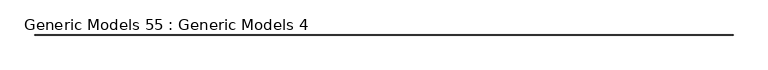
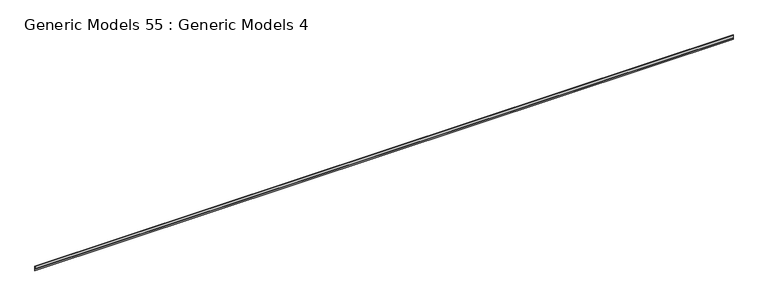
"""IFC4 building model written with IfcOpenShell, lengths in millimetres: proxy geometry, Generic Models 55 : Generic Models 4."""

from ifc_helpers import new_model, si_unit, frame, origin, place, context, project, spatial, polyline, outline, extrude, source, transform, mapped, element, save


def generic_models_55_generic_models_4_dafe8dc5(model_context):
    return source(origin(), model_context, "Body", "SweptSolid", [
        extrude(outline(polyline([(11501.3557472, 129460.23396), (11501.3557472, 129538.225544), (11502.1494972, 129538.225544), (11502.1494972, 129460.3739195), (11506.1872906, 129449.2801733), (11506.1872906, 129411.3880757), (11505.3935406, 129411.3880757), (11505.3935406, 129449.1402137), (11501.3557472, 129460.23396)])), frame((-14733.8627414, 0.0, 0.0), z_axis=(1.0, 0.0, 0.0), x_axis=(0.0, 1.0, 0.0)), (0.0, 0.0, 1.0), 18643.6),
    ])


if __name__ == "__main__":
    model = new_model("IFC4")
    model_context = context("Model", 3, world=origin())
    ifc_project = project(units=[si_unit("LENGTHUNIT", "METRE", prefix="MILLI")], contexts=[model_context])
    site = spatial("IfcSite", under=ifc_project)
    building = spatial("IfcBuilding", under=site)
    placement = place(None, origin())
    generic_models_55_generic_models_4_shape = generic_models_55_generic_models_4_dafe8dc5(model_context)
    element("IfcBuildingElementProxy", 1, Name="Generic Models 55 : Generic Models 4", ObjectType="Generic Models 55 : Generic Models 4", at=placement, inside=building, context=model_context, shape_type="MappedRepresentation", body=[
        mapped(generic_models_55_generic_models_4_shape, transform((0.0, 0.0, 0.0), x_axis=(1.0, 0.0, 0.0), y_axis=(0.0, 1.0, 0.0), z_axis=(0.0, 0.0, 1.0))),
    ])
    save(model, "model.ifc")

# Revit data of these elements
# Element 1 (IfcBuildingElementProxy, "Generic Models 55 : Generic Models 4")
#   Materials on its faces: "_(2) LAYERS NO. 30 ASTM D226 ASPHALT SATURATED ORGANIC FELT"
# Materials
#   "_(2) LAYERS NO. 30 ASTM D226 ASPHALT SATURATED ORGANIC FELT": class "Generic", colour RGB 67 154 161, transparency 0, Cost = 0
